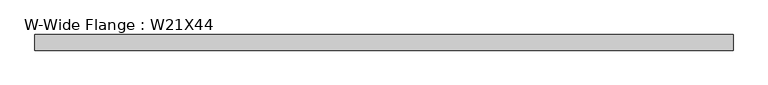
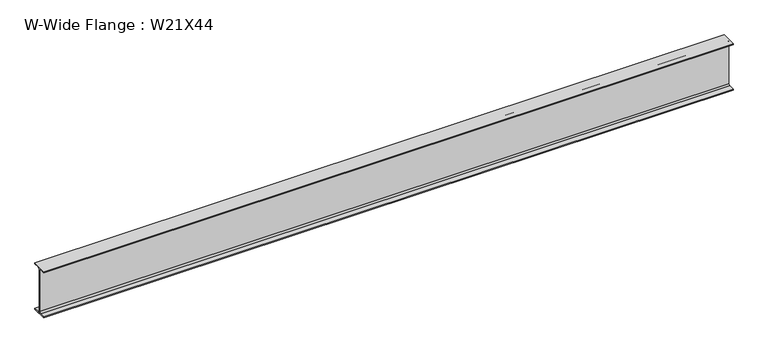
"""IFC4 building model written with IfcOpenShell, lengths in millimetres: beam geometry, W-Wide Flange : W21X44."""

from ifc_helpers import new_model, si_unit, point, frame, frame_2d, origin, place, context, project, spatial, polyline, circle_curve, trimmed, segment, composite_curve, outline, extrude, source, transform, mapped, element, save


def w_wide_flange_w21x44_417b1038(model_context):
    return source(origin(), model_context, "Body", "SweptSolid", [
        extrude(outline(composite_curve([segment(polyline([(82.55, -251.46), (82.55, -262.89), (-82.55, -262.89), (-82.55, -251.46), (-21.59, -251.46)]), True, "CONTINUOUS"), segment(trimmed(circle_curve(frame_2d((-21.59, -234.315)), 17.145), [point((-21.59, -251.46))], [point((-4.445, -234.315))], True, "CARTESIAN"), True, "CONTINUOUS"), segment(polyline([(-4.445, -234.315), (-4.445, 234.315)]), True, "CONTINUOUS"), segment(trimmed(circle_curve(frame_2d((-21.59, 234.315)), 17.145), [point((-4.445, 234.315))], [point((-21.59, 251.46))], True, "CARTESIAN"), True, "CONTINUOUS"), segment(polyline([(-21.59, 251.46), (-82.55, 251.46), (-82.55, 262.89), (82.55, 262.89), (82.55, 251.46), (21.59, 251.46)]), True, "CONTINUOUS"), segment(trimmed(circle_curve(frame_2d((21.59, 234.315)), 17.145), [point((21.59, 251.46))], [point((4.445, 234.315))], True, "CARTESIAN"), True, "CONTINUOUS"), segment(polyline([(4.445, 234.315), (4.445, -234.315)]), True, "CONTINUOUS"), segment(trimmed(circle_curve(frame_2d((21.59, -234.315)), 17.145), [point((4.445, -234.315))], [point((21.59, -251.46))], True, "CARTESIAN"), True, "CONTINUOUS"), segment(polyline([(21.59, -251.46), (82.55, -251.46)]), True, "CONTINUOUS")], self_intersect=False)), frame((-3654.3753906, 0.0, 0.0), z_axis=(1.0, 0.0, 0.0), x_axis=(0.0, 1.0, 0.0)), (0.0, 0.0, 1.0), 7377.8566406),
    ])


if __name__ == "__main__":
    model = new_model("IFC4")
    model_context = context("Model", 3, world=origin())
    ifc_project = project(units=[si_unit("LENGTHUNIT", "METRE", prefix="MILLI")], contexts=[model_context])
    site = spatial("IfcSite", under=ifc_project)
    building = spatial("IfcBuilding", under=site)
    placement = place(None, origin())
    w_wide_flange_w21x44_shape = w_wide_flange_w21x44_417b1038(model_context)
    element("IfcBeam", 1, ObjectType="W-Wide Flange : W21X44", at=placement, inside=building, context=model_context, shape_type="MappedRepresentation", body=[
        mapped(w_wide_flange_w21x44_shape, transform((0.0, 0.0, 0.0), x_axis=(1.0, 0.0, 0.0), y_axis=(0.0, 1.0, 0.0), z_axis=(0.0, 0.0, 1.0))),
    ])
    save(model, "model.ifc")

# Revit data of these elements
# Type "W-Wide Flange : W21X44"
#   Assembly Code = "B10"
#   W = 44
#   Length [instance default] = 1524 mm
#   bf = 165.1 mm
#   d = 525.78 mm
#   k = 28.575 mm
#   k2 = 17.145 mm
#   tf = 11.43 mm
#   tw = 8.89 mm
#   A = 0.00838708 m²
#   Structural Material [instance default] = Steel ASTM A992
# Element 1 (IfcBeam, "W-Wide Flange : W21X44")
#   Structural Material = Aluminum, Anodized Red
#   Materials on its faces: "Aluminum, Anodized Red"
# Materials
#   "Steel ASTM A992": class "Metal", colour RGB 128 0 0, transparency 0, Description = "Structural steel 50ksi", Cost = 0
#   "Aluminum, Anodized Red": class "Metal", colour RGB 120 120 120, transparency 0, Description = "Anodized aluminum, red", Cost = 0
